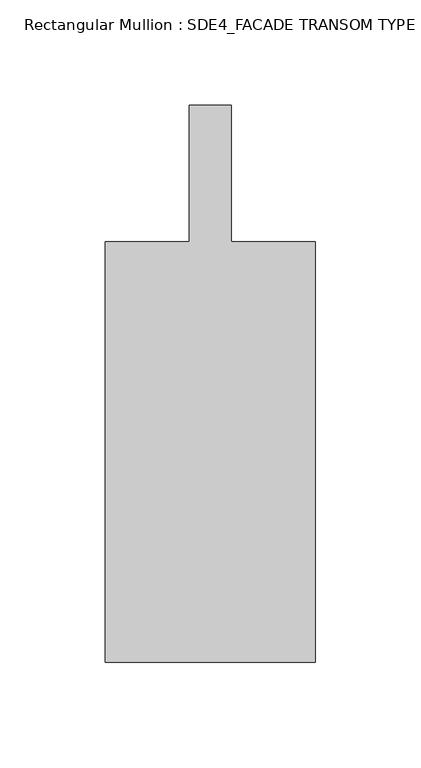
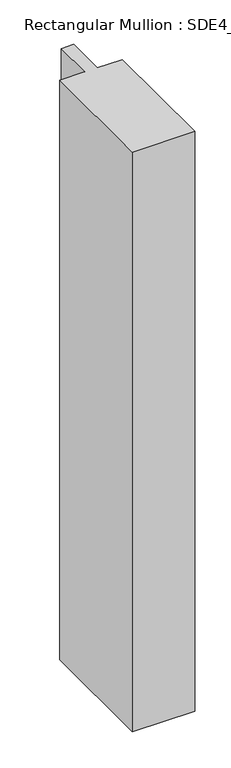
"""IFC4 building model written with IfcOpenShell, lengths in millimetres: member geometry, Rectangular Mullion : SDE4_FACADE TRANSOM TYPE 2."""

from ifc_helpers import new_model, si_unit, frame, origin, place, context, project, spatial, polyline, outline, extrude, source, transform, mapped, element, save


def rectangular_mullion_sde4_facade_transom_type_2_c3f0b787(model_context):
    return source(origin(), model_context, "Body", "SweptSolid", [
        extrude(outline(polyline([(50.0, -132.5), (-50.0, -132.5), (-50.0, 67.5), (-10.0, 67.5), (-10.0, 132.5), (10.0, 132.5), (10.0, 67.5), (50.0, 67.5), (50.0, -132.5)])), frame((0.0, 0.0, -978.0), z_axis=(0.0, 0.0, 1.0), x_axis=(1.0, 0.0, 0.0)), (0.0, 0.0, 1.0), 978.0),
    ])


if __name__ == "__main__":
    model = new_model("IFC4")
    model_context = context("Model", 3, world=origin())
    ifc_project = project(units=[si_unit("LENGTHUNIT", "METRE", prefix="MILLI")], contexts=[model_context])
    site = spatial("IfcSite", under=ifc_project)
    building = spatial("IfcBuilding", under=site)
    placement = place(None, origin())
    rectangular_mullion_sde4_facade_transom_type_2_shape = rectangular_mullion_sde4_facade_transom_type_2_c3f0b787(model_context)
    element("IfcMember", 1, ObjectType="Rectangular Mullion : SDE4_FACADE TRANSOM TYPE 2", at=placement, inside=building, context=model_context, shape_type="MappedRepresentation", body=[
        mapped(rectangular_mullion_sde4_facade_transom_type_2_shape, transform((0.0, 0.0, 0.0), x_axis=(1.0, 0.0, 0.0), y_axis=(0.0, 1.0, 0.0), z_axis=(0.0, 0.0, 1.0))),
    ])
    save(model, "model.ifc")

# Revit data of these elements
# Type "Rectangular Mullion : SDE4_FACADE TRANSOM TYPE 2"
#   built-in parameter 1007322 = 0.869423 (stored number, unit not read)
#   built-in parameter 1007321 = 0.164042 (stored number, unit not read)
#   built-in parameter 1007320 = 0.164042 (stored number, unit not read)
